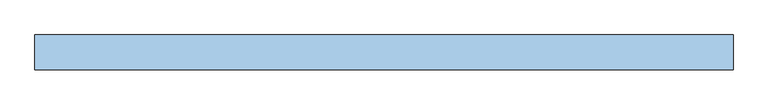
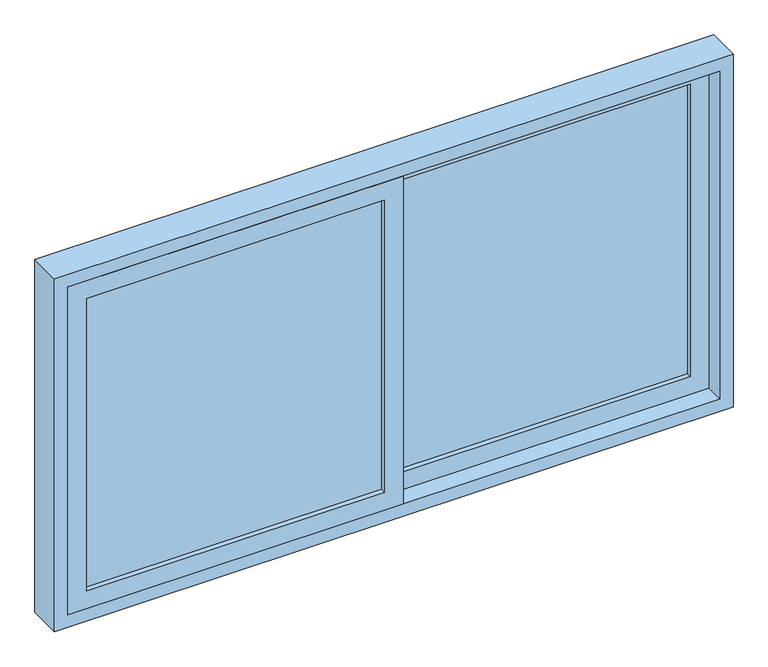
"""IFC4 building model written with IfcOpenShell, lengths in millimetres: window geometry, Janela de correr - 2 Painéis : Janela de correr - 2 Painéis."""

from ifc_helpers import new_model, si_unit, frame, origin, place, context, project, spatial, polyline, outline, extrude, source, transform, mapped, element, save


def window_c3c1e9cb(model_context):
    return source(origin(), model_context, "Body", "SweptSolid", [
        extrude(outline(polyline([(685.0, -25.0), (685.0, 865.0), (1605.0, 865.0), (1605.0, -25.0), (685.0, -25.0)]), holes=[polyline([(1555.0, 25.0), (1555.0, 815.0), (735.0, 815.0), (735.0, 25.0), (1555.0, 25.0)])]), frame((0.0, -20.0, 0.0), z_axis=(0.0, 1.0, 0.0), x_axis=(0.0, 0.0, 1.0)), (0.0, 0.0, 1.0), 40.0),
        extrude(outline(polyline([(1605.0, 25.0), (1605.0, -865.0), (685.0, -865.0), (685.0, 25.0), (1605.0, 25.0)]), holes=[polyline([(735.0, -25.0), (735.0, -815.0), (1555.0, -815.0), (1555.0, -25.0), (735.0, -25.0)])]), frame((0.0, -70.0, 0.0), z_axis=(0.0, 1.0, 0.0), x_axis=(0.0, 0.0, 1.0)), (0.0, 0.0, 1.0), 40.0),
        extrude(outline(polyline([(1640.0, 900.0), (1640.0, -900.0), (650.0, -900.0), (650.0, 900.0), (1640.0, 900.0)]), holes=[polyline([(685.0, 865.0), (685.0, -865.0), (1605.0, -865.0), (1605.0, 865.0), (685.0, 865.0)])]), frame((0.0, -70.0, 0.0), z_axis=(0.0, 1.0, 0.0), x_axis=(0.0, 0.0, 1.0)), (0.0, 0.0, 1.0), 90.0),
        extrude(outline(polyline([(25.0, 7.0), (815.0, 7.0), (815.0, -7.0), (25.0, -7.0), (25.0, 7.0)])), frame((0.0, 0.0, 735.0), z_axis=(0.0, 0.0, 1.0), x_axis=(1.0, 0.0, 0.0)), (0.0, 0.0, 1.0), 820.0),
        extrude(outline(polyline([(-815.0, -43.0), (-25.0, -43.0), (-25.0, -57.0), (-815.0, -57.0), (-815.0, -43.0)])), frame((0.0, 0.0, 735.0), z_axis=(0.0, 0.0, 1.0), x_axis=(1.0, 0.0, 0.0)), (0.0, 0.0, 1.0), 820.0),
    ])


if __name__ == "__main__":
    model = new_model("IFC4")
    model_context = context("Model", 3, world=origin())
    ifc_project = project(units=[si_unit("LENGTHUNIT", "METRE", prefix="MILLI")], contexts=[model_context])
    site = spatial("IfcSite", under=ifc_project)
    building = spatial("IfcBuilding", under=site)
    placement = place(None, origin())
    window_shape = window_c3c1e9cb(model_context)
    element("IfcWindow", 1, ObjectType="Janela de correr - 2 Painéis : Janela de correr - 2 Painéis", at=placement, inside=building, context=model_context, shape_type="MappedRepresentation", body=[
        mapped(window_shape, transform((0.0, 0.0, 0.0), x_axis=(1.0, 0.0, 0.0), y_axis=(0.0, 1.0, 0.0), z_axis=(0.0, 0.0, 1.0))),
    ])
    save(model, "model.ifc")

# Revit data of these elements
# Type "Janela de correr - 2 Painéis : Janela de correr - 2 Painéis"
#   Type Mark = "EF27"
#   Construction Type Id = "GSP4R"
#   Analytic Construction = "Vidraça única Pilkington 1/8 pol"
#   Visual Light Transmittance = 0.9
#   Solar Heat Gain Coefficient = 0.78
#   Rough Width = 1.800 m
#   Rough Height = 0.990 m
#   Largura da moldura do painel = 0.050 m
#   Espessura da moldura do painel = 0.040 m
#   Height = 0.990 m
#   Heat Transfer Coefficient (U) = 3.6886 W/(m²·K)
#   Largura da estrutura = 0.035 m
#   Espessura da moldura = 0.090 m
#   Altura-padrão do peitoril = 0.650 m
#   Width = 1.800 m
#   Define Thermal Properties by = 1
#   Vidro = none
#   Material da moldura = none
#   Wall Closure = (empty or 0)
# Element 1 (IfcWindow, "Janela de correr - 2 Painéis : Janela de correr - 2 Painéis")
#   Materials on its faces: "Glass"
# Materials
#   "Glass": class "Glass", colour RGB 0 128 192, transparency 0.75, Description = "Soda Lime Glass", Cost = 0
